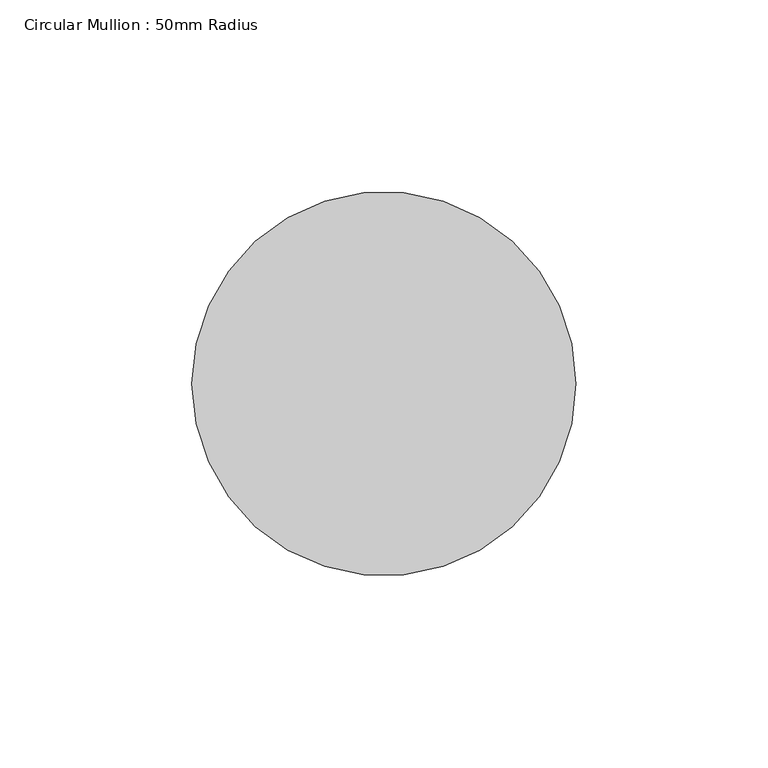
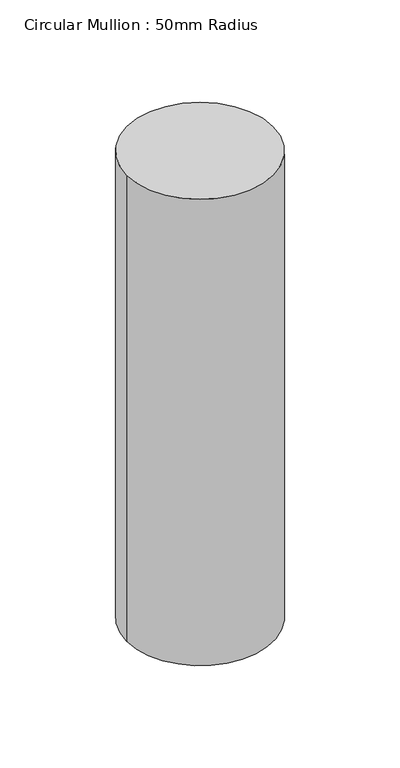
"""IFC4 building model written with IfcOpenShell, lengths in millimetres: member geometry, Circular Mullion : 50mm Radius."""

import ifcopenshell
import ifcopenshell.guid

model = None  # the IFC model being written
_history = None  # IfcOwnerHistory: only IFC2X3 demands one
_inside = {}  # id of a spatial element -> (the spatial element, [elements in it])
_under = {}  # id of a project, library or spatial element -> (it, [spatial elements below it])
_declared = {}  # id of a project -> (the project, [libraries it declares])
_typed = {}  # id of a type object -> (the type object, [elements of that type])
_made_of = {}  # id of a material, layer set ... -> (it, [elements and type objects made of it])


def new_model(schema):
    """Start an empty IFC model of exactly this schema.

    Asked for "IFC4X3", IfcOpenShell would pick the latest addendum, in which some entities
    have other attributes; the version numbers below select the first issue.
    IFC2X3 requires an IfcOwnerHistory on every rooted entity: one is made here for all.
    """
    global model, _history
    if schema == "IFC4X3":
        model = ifcopenshell.file(schema_version=(4, 3, 0, 0))
    else:
        model = ifcopenshell.file(schema=schema)
    _inside.clear()
    _under.clear()
    _declared.clear()
    _typed.clear()
    _made_of.clear()
    _history = None
    if model.schema == "IFC2X3":
        org = make("IfcOrganization", Name="unknown")
        user = make(
            "IfcPersonAndOrganization",
            ThePerson=make("IfcPerson", FamilyName="unknown"),
            TheOrganization=org,
        )
        app = make(
            "IfcApplication",
            ApplicationDeveloper=org,
            Version="unknown",
            ApplicationFullName="unknown",
            ApplicationIdentifier="unknown",
        )
        _history = make(
            "IfcOwnerHistory",
            OwningUser=user,
            OwningApplication=app,
            ChangeAction="ADDED",
            CreationDate=0,
        )
    return model


def make(cls, **values):
    """One entity of the class cls with the attributes given. An attribute that is None is left unset."""
    return model.create_entity(
        cls, **{name: value for name, value in values.items() if value is not None}
    )


def rooted(cls, **values):
    """An entity with a GlobalId (a new one), such as an element, a storey or a relation."""
    return make(cls, GlobalId=ifcopenshell.guid.new(), OwnerHistory=_history, **values)


def si_unit(unit_type, name, prefix=None):
    """IfcSIUnit, for example si_unit("LENGTHUNIT", "METRE", prefix="MILLI")."""
    return make("IfcSIUnit", UnitType=unit_type, Prefix=prefix, Name=name)


def assignment(units):
    """IfcUnitAssignment: the units of a project."""
    return None if units is None else make("IfcUnitAssignment", Units=units)


def point(xyz):
    """IfcCartesianPoint."""
    return None if xyz is None else make("IfcCartesianPoint", Coordinates=xyz)


def direction(xyz):
    """IfcDirection."""
    return None if xyz is None else make("IfcDirection", DirectionRatios=xyz)


def frame(location, z_axis=None, x_axis=None):
    """IfcAxis2Placement3D, a coordinate frame: its origin and axes. An axis left out is left unset."""
    return make(
        "IfcAxis2Placement3D",
        Location=point(location),
        Axis=direction(z_axis),
        RefDirection=direction(x_axis),
    )


def frame_2d(location, x_axis=None):
    """IfcAxis2Placement2D, a coordinate frame in the plane: its origin and x axis."""
    return make(
        "IfcAxis2Placement2D", Location=point(location), RefDirection=direction(x_axis)
    )


def origin():
    """The frame at (0, 0, 0) with its axes left unset."""
    return frame((0.0, 0.0, 0.0))


def origin_2d():
    """The frame at (0, 0) in the plane with its x axis left unset."""
    return frame_2d((0.0, 0.0))


def place(relative_to, where):
    """IfcLocalPlacement: puts the frame where relative to a parent placement (None: the world)."""
    return make(
        "IfcLocalPlacement", PlacementRelTo=relative_to, RelativePlacement=where
    )


def context(
    kind, dimensions, precision=None, world=None, true_north=None, identifier=None
):
    """IfcGeometricRepresentationContext, for example the 3D "Model" context."""
    return make(
        "IfcGeometricRepresentationContext",
        ContextIdentifier=identifier,
        ContextType=kind,
        CoordinateSpaceDimension=dimensions,
        Precision=precision,
        WorldCoordinateSystem=world,
        TrueNorth=true_north,
    )


def project(units=None, contexts=None):
    """IfcProject with its units and contexts."""
    return rooted(
        "IfcProject",
        Name="project",
        RepresentationContexts=contexts,
        UnitsInContext=assignment(units),
    )


def spatial(cls, under=None, at=None, **own):
    """A site, building, storey or space (cls), placed at a placement, below another one or the project."""
    s = rooted(cls, ObjectPlacement=at, **own)
    if under is not None:
        _under.setdefault(under.id(), (under, []))[1].append(s)
    return s


def circle_curve(where, radius):
    """IfcCircle in the frame where."""
    return make("IfcCircle", Position=where, Radius=radius)


def trimmed(basis, trim1, trim2, sense, master):
    """IfcTrimmedCurve: the piece of a basis curve between two trims."""
    return make(
        "IfcTrimmedCurve",
        BasisCurve=basis,
        Trim1=trim1,
        Trim2=trim2,
        SenseAgreement=sense,
        MasterRepresentation=master,
    )


def segment(curve, same_sense, transition):
    """IfcCompositeCurveSegment."""
    return make(
        "IfcCompositeCurveSegment",
        Transition=transition,
        SameSense=same_sense,
        ParentCurve=curve,
    )


def composite_curve(segments, self_intersect=None):
    """IfcCompositeCurve: segments joined end to end."""
    return make("IfcCompositeCurve", Segments=segments, SelfIntersect=self_intersect)


def outline(outer, holes=None, kind="AREA"):
    """IfcArbitraryClosedProfileDef: a profile drawn as a closed curve; with holes, ...WithVoids."""
    if holes is None:
        return make("IfcArbitraryClosedProfileDef", ProfileType=kind, OuterCurve=outer)
    return make(
        "IfcArbitraryProfileDefWithVoids",
        ProfileType=kind,
        OuterCurve=outer,
        InnerCurves=holes,
    )


def extrude(swept, where, along, depth):
    """IfcExtrudedAreaSolid: the profile swept, set in the frame where, extruded along a direction by depth."""
    return make(
        "IfcExtrudedAreaSolid",
        SweptArea=swept,
        Position=where,
        ExtrudedDirection=direction(along),
        Depth=depth,
    )


def shape(context_of_items, identifier, shape_type, items):
    """IfcShapeRepresentation: the items that make up one representation, for example the "Body"."""
    return make(
        "IfcShapeRepresentation",
        ContextOfItems=context_of_items,
        RepresentationIdentifier=identifier,
        RepresentationType=shape_type,
        Items=items,
    )


def source(mapping_origin, context_of_items, identifier, shape_type, items):
    """IfcRepresentationMap: a shape defined once, which mapped items show again and again."""
    return make(
        "IfcRepresentationMap",
        MappingOrigin=mapping_origin,
        MappedRepresentation=shape(context_of_items, identifier, shape_type, items),
    )


def transform(
    local_origin,
    x_axis=None,
    y_axis=None,
    z_axis=None,
    scale=None,
    scale2=None,
    scale3=None,
    uniform=True,
):
    """IfcCartesianTransformationOperator3D, or its non-uniform kind. x_axis, y_axis, z_axis: its Axis1, 2, 3."""
    if uniform:
        return make(
            "IfcCartesianTransformationOperator3D",
            Axis1=direction(x_axis),
            Axis2=direction(y_axis),
            LocalOrigin=point(local_origin),
            Scale=scale,
            Axis3=direction(z_axis),
        )
    return make(
        "IfcCartesianTransformationOperator3DnonUniform",
        Axis1=direction(x_axis),
        Axis2=direction(y_axis),
        LocalOrigin=point(local_origin),
        Scale=scale,
        Axis3=direction(z_axis),
        Scale2=scale2,
        Scale3=scale3,
    )


def mapped(mapping_source, mapping_target):
    """IfcMappedItem: shows the shape of a source again, moved by a transform."""
    return make(
        "IfcMappedItem", MappingSource=mapping_source, MappingTarget=mapping_target
    )


def made_of(thing, what):
    """Note that an element or type object is made of a material, layer set ...; save() writes the relation."""
    if what is not None:
        _made_of.setdefault(what.id(), (what, []))[1].append(thing)
    return thing


def element(
    cls,
    number,
    at=None,
    inside=None,
    cuts=None,
    type_object=None,
    material=None,
    context=None,
    identifier="Body",
    shape_type=None,
    held_by="IfcProductDefinitionShape",
    body=None,
    shapes=None,
    **own,
):
    """One element of the class cls, such as IfcWall. Its Tag is "e" and its number.

    at: its placement. inside: the storey or other place that contains it. cuts: it is an
    opening in that element (IfcRelVoidsElement). A single representation is given by context,
    identifier, shape_type and body (its items); several are given by shapes. held_by: the class
    of the entity that holds the representations. save() writes the other relations.
    """
    e = rooted(cls, Tag="e%d" % number, ObjectPlacement=at, **own)
    if body is not None:
        shapes = [shape(context, identifier, shape_type, body)]
    if shapes is not None:
        e.Representation = make(held_by, Representations=shapes)
    if inside is not None:
        _inside.setdefault(inside.id(), (inside, []))[1].append(e)
    if cuts is not None:
        rooted(
            "IfcRelVoidsElement", RelatingBuildingElement=cuts, RelatedOpeningElement=e
        )
    if type_object is not None:
        _typed.setdefault(type_object.id(), (type_object, []))[1].append(e)
    return made_of(e, material)


def aggregate(whole, parts):
    """IfcRelAggregates: a whole, such as a stair, and the parts it consists of."""
    return rooted("IfcRelAggregates", RelatingObject=whole, RelatedObjects=parts)


def save(model, path):
    """Write the relations noted so far, then the file.

    IfcRelAggregates (storeys below a building ...), IfcRelContainedInSpatialStructure (elements
    in a storey), IfcRelDefinesByType, IfcRelAssociatesMaterial and IfcRelDeclares: one each for
    every whole, place, type object, material and project.
    """
    for whole, parts in _under.values():
        aggregate(whole, parts)
    for where, things in _inside.values():
        rooted(
            "IfcRelContainedInSpatialStructure",
            RelatedElements=things,
            RelatingStructure=where,
        )
    for kind, things in _typed.values():
        rooted("IfcRelDefinesByType", RelatedObjects=things, RelatingType=kind)
    for what, things in _made_of.values():
        rooted("IfcRelAssociatesMaterial", RelatedObjects=things, RelatingMaterial=what)
    for by, libraries in _declared.values():
        rooted("IfcRelDeclares", RelatingContext=by, RelatedDefinitions=libraries)
    model.write(path)


def circular_mullion_50mm_radius_90580c94(model_context):
    return source(origin(), model_context, "Body", "SweptSolid", [
        extrude(outline(composite_curve([segment(trimmed(circle_curve(origin_2d(), 50.0), [point((50.0, 0.0))], [point((-50.0, 0.0))], False, "CARTESIAN"), True, "CONTINUOUS"), segment(trimmed(circle_curve(origin_2d(), 50.0), [point((-50.0, 0.0))], [point((50.0, 0.0))], False, "CARTESIAN"), True, "CONTINUOUS")], self_intersect=False)), frame((0.0, 0.0, -336.2636025), z_axis=(0.0, 0.0, 1.0), x_axis=(1.0, 0.0, 0.0)), (0.0, 0.0, 1.0), 336.2636025),
    ])


if __name__ == "__main__":
    model = new_model("IFC4")
    model_context = context("Model", 3, world=origin())
    ifc_project = project(units=[si_unit("LENGTHUNIT", "METRE", prefix="MILLI")], contexts=[model_context])
    site = spatial("IfcSite", under=ifc_project)
    building = spatial("IfcBuilding", under=site)
    placement = place(None, origin())
    circular_mullion_50mm_radius_shape = circular_mullion_50mm_radius_90580c94(model_context)
    element("IfcMember", 1, ObjectType="Circular Mullion : 50mm Radius", at=placement, inside=building, context=model_context, shape_type="MappedRepresentation", body=[
        mapped(circular_mullion_50mm_radius_shape, transform((0.0, 0.0, 0.0), x_axis=(1.0, 0.0, 0.0), y_axis=(0.0, 1.0, 0.0), z_axis=(0.0, 0.0, 1.0))),
    ])
    save(model, "model.ifc")

# Revit data of these elements
# Type "Circular Mullion : 50mm Radius"
#   built-in parameter 1007350 = 0.164042 (stored number, unit not read)
# Element 1 (IfcMember, "Circular Mullion : 50mm Radius")
#   Materials on its faces: "Aluminium"
# Materials
#   "Aluminium": class "Metal", colour RGB 247 247 247, transparency 0, Description = "Aluminium 6061", Cost = 0
